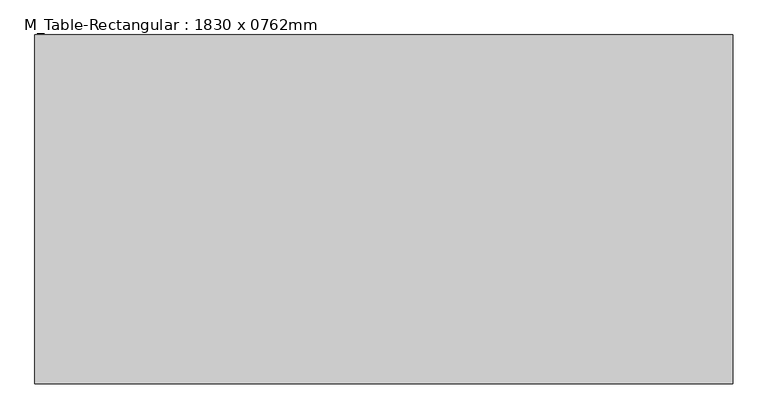
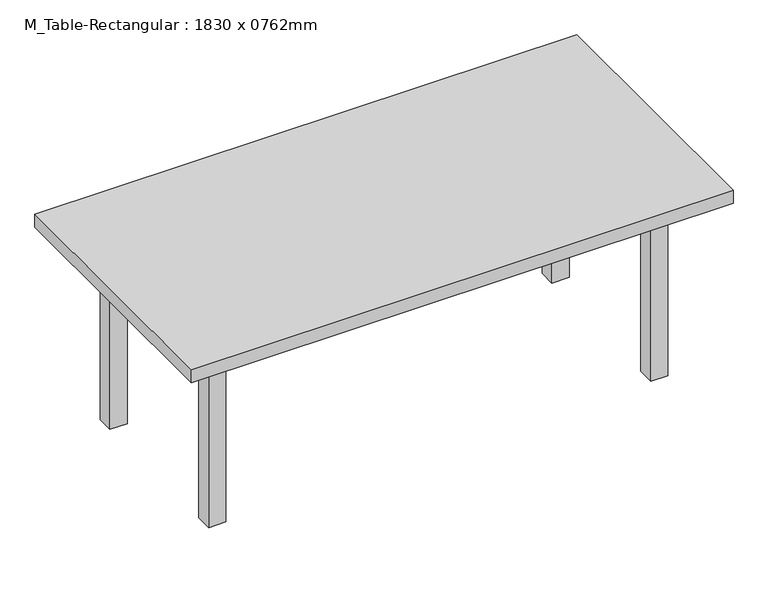
"""IFC4 building model written with IfcOpenShell, lengths in millimetres: furniture geometry, M_Table-Rectangular : 1830 x 0762mm."""

from ifc_helpers import new_model, si_unit, frame, origin, origin_with_axes, place, context, project, spatial, polyline, outline, extrude, source, transform, mapped, element, save


def m_table_rectangular_1830_x_0762mm_34bc21c2(model_context):
    return source(origin(), model_context, "Body", "SweptSolid", [
        extrude(outline(polyline([(784.1, 309.5), (784.1, 284.1), (-784.1, 284.1), (-784.1, 309.5), (784.1, 309.5)])), frame((0.0, 0.0, 609.6), z_axis=(0.0, 0.0, 1.0), x_axis=(1.0, 0.0, 0.0)), (0.0, 0.0, 1.0), 101.6),
        extrude(outline(polyline([(784.1, -309.5), (-784.1, -309.5), (-784.1, -284.1), (784.1, -284.1), (784.1, -309.5)])), frame((0.0, 0.0, 609.6), z_axis=(0.0, 0.0, 1.0), x_axis=(1.0, 0.0, 0.0)), (0.0, 0.0, 1.0), 101.6),
        extrude(outline(polyline([(-796.8, -284.1), (-822.2, -284.1), (-822.2, 284.1), (-796.8, 284.1), (-796.8, -284.1)])), frame((0.0, 0.0, 609.6), z_axis=(0.0, 0.0, 1.0), x_axis=(1.0, 0.0, 0.0)), (0.0, 0.0, 1.0), 101.6),
        extrude(outline(polyline([(796.8, -284.1), (796.8, 284.1), (822.2, 284.1), (822.2, -284.1), (796.8, -284.1)])), frame((0.0, 0.0, 609.6), z_axis=(0.0, 0.0, 1.0), x_axis=(1.0, 0.0, 0.0)), (0.0, 0.0, 1.0), 101.6),
        extrude(outline(polyline([(1000.0, 500.0), (1000.0, -500.0), (-1000.0, -500.0), (-1000.0, 500.0), (1000.0, 500.0)])), frame((0.0, 0.0, 711.2), z_axis=(0.0, 0.0, 1.0), x_axis=(1.0, 0.0, 0.0)), (0.0, 0.0, 1.0), 50.8),
        extrude(outline(polyline([(-784.1, 347.6), (-784.1, 284.1), (-847.6, 284.1), (-847.6, 347.6), (-784.1, 347.6)])), origin_with_axes(), (0.0, 0.0, 1.0), 711.2),
        extrude(outline(polyline([(784.1, 347.6), (847.6, 347.6), (847.6, 284.1), (784.1, 284.1), (784.1, 347.6)])), origin_with_axes(), (0.0, 0.0, 1.0), 711.2),
        extrude(outline(polyline([(-784.1, -347.6), (-847.6, -347.6), (-847.6, -284.1), (-784.1, -284.1), (-784.1, -347.6)])), origin_with_axes(), (0.0, 0.0, 1.0), 711.2),
        extrude(outline(polyline([(784.1, -347.6), (784.1, -284.1), (847.6, -284.1), (847.6, -347.6), (784.1, -347.6)])), origin_with_axes(), (0.0, 0.0, 1.0), 711.2),
    ])


if __name__ == "__main__":
    model = new_model("IFC4")
    model_context = context("Model", 3, world=origin())
    ifc_project = project(units=[si_unit("LENGTHUNIT", "METRE", prefix="MILLI")], contexts=[model_context])
    site = spatial("IfcSite", under=ifc_project)
    building = spatial("IfcBuilding", under=site)
    placement = place(None, origin())
    m_table_rectangular_1830_x_0762mm_shape = m_table_rectangular_1830_x_0762mm_34bc21c2(model_context)
    element("IfcFurniture", 1, ObjectType="M_Table-Rectangular : 1830 x 0762mm", at=placement, inside=building, context=model_context, shape_type="MappedRepresentation", body=[
        mapped(m_table_rectangular_1830_x_0762mm_shape, transform((0.0, 0.0, 0.0), x_axis=(1.0, 0.0, 0.0), y_axis=(0.0, 1.0, 0.0), z_axis=(0.0, 0.0, 1.0))),
    ])
    save(model, "model.ifc")

# Revit data of these elements
# Type "M_Table-Rectangular : 1830 x 0762mm"
#   Height = 0.762 m
#   Length = 2.00 m
#   Width = 1.00 m
#   Base Material = Birch
#   Top Material = Birch
#   Default Elevation = 0
# Element 1 (IfcFurniture, "M_Table-Rectangular : 1830 x 0762mm")
#   Materials on its faces: "Birch"
# Materials
#   "Birch": class "Wood", colour RGB 224 178 126, transparency 0, Description = "Betula Alleghaniensis", Cost = 0
